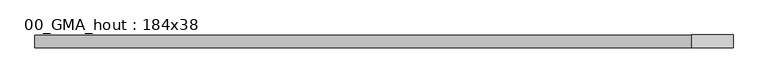
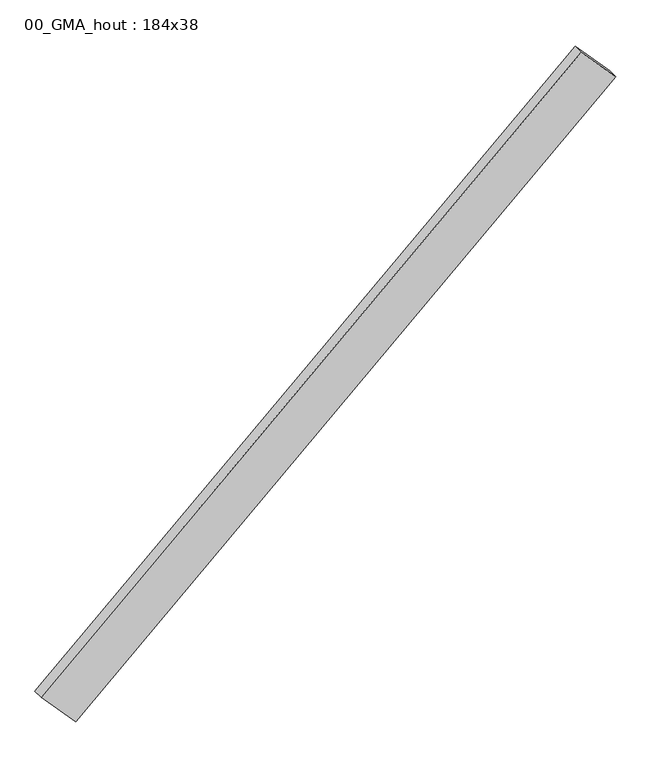
"""IFC4 building model written with IfcOpenShell, lengths in millimetres: proxy geometry, 00_GMA_hout : 184x38."""

from ifc_helpers import new_model, si_unit, frame, origin, place, context, project, spatial, polyline, outline, extrude, source, transform, mapped, element, save


def proxy_00_gma_hout_184x38_1d2382f2(model_context):
    return source(origin(), model_context, "Body", "SweptSolid", [
        extrude(outline(polyline([(-19.0, 0.0), (19.0, 0.0), (19.0, -2617.0000001), (-19.0, -2617.0000001), (-19.0, 0.0)])), frame((-400.2270235, 19.0, -613.6855812), z_axis=(-0.67357883778224, 0.0, 0.7391153829355245), x_axis=(0.0, 1.0, 0.0)), (0.0, 0.0, 1.0), 184.0),
    ])


if __name__ == "__main__":
    model = new_model("IFC4")
    model_context = context("Model", 3, world=origin())
    ifc_project = project(units=[si_unit("LENGTHUNIT", "METRE", prefix="MILLI")], contexts=[model_context])
    site = spatial("IfcSite", under=ifc_project)
    building = spatial("IfcBuilding", under=site)
    placement = place(None, origin())
    proxy_00_gma_hout_184x38_shape = proxy_00_gma_hout_184x38_1d2382f2(model_context)
    element("IfcBuildingElementProxy", 1, Name="00_GMA_hout : 184x38", ObjectType="00_GMA_hout : 184x38", at=placement, inside=building, context=model_context, shape_type="MappedRepresentation", body=[
        mapped(proxy_00_gma_hout_184x38_shape, transform((0.0, 0.0, 0.0), x_axis=(1.0, 0.0, 0.0), y_axis=(0.0, 1.0, 0.0), z_axis=(0.0, 0.0, 1.0))),
    ])
    save(model, "model.ifc")

# Revit data of these elements
# Type "00_GMA_hout : 184x38"
#   lengte [instance default] = 1198.641 mm
#   h = 38 mm
#   b = 184 mm
#   materiaal = 00_hout_vuren_generiek
#   PositionProfile [instance default] = 00_GMP_rectangle : TopLeft
#   Default Elevation = 0
# Element 1 (IfcBuildingElementProxy, "00_GMA_hout : 184x38")
#   lengte = 2617 mm
#   PositionProfile = 00_GMP_rectangle : TopRight
#   Materials on its faces: "00_hout_vuren_generiek"
# Materials
#   "00_hout_vuren_generiek": class "Wood", colour RGB 255 128 0, transparency 0, Manufacturer = "RevitGG", URL = "www.revitgg.nl", Description = "Hout, vuren, generiek", Cost = 0
